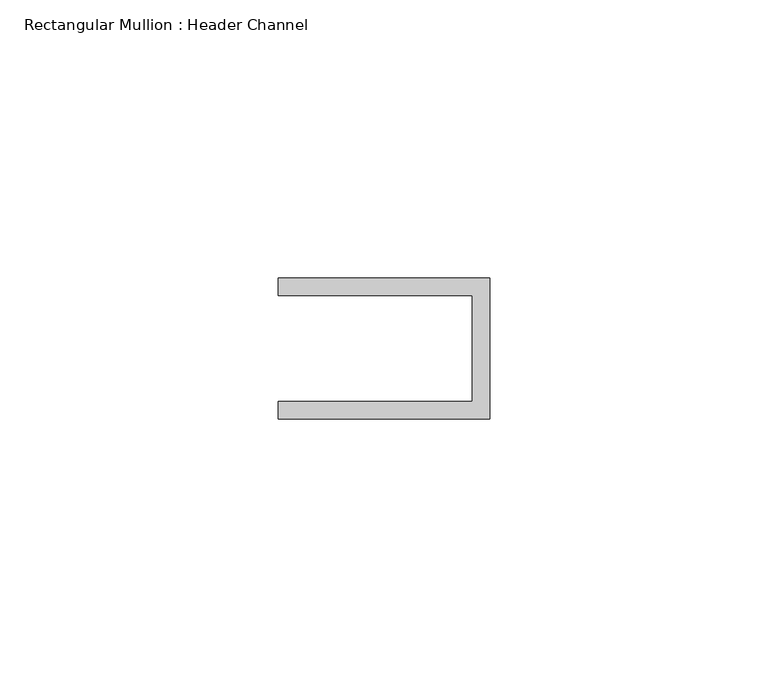
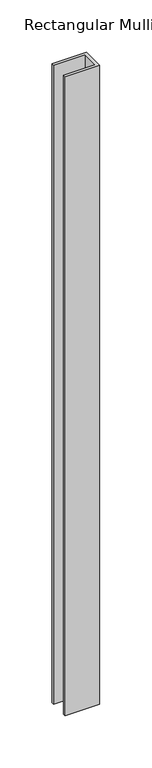
"""IFC4 building model written with IfcOpenShell, lengths in millimetres: member geometry, Rectangular Mullion : Header Channel."""

import ifcopenshell
import ifcopenshell.guid

model = None  # the IFC model being written
_history = None  # IfcOwnerHistory: only IFC2X3 demands one
_inside = {}  # id of a spatial element -> (the spatial element, [elements in it])
_under = {}  # id of a project, library or spatial element -> (it, [spatial elements below it])
_declared = {}  # id of a project -> (the project, [libraries it declares])
_typed = {}  # id of a type object -> (the type object, [elements of that type])
_made_of = {}  # id of a material, layer set ... -> (it, [elements and type objects made of it])


def new_model(schema):
    """Start an empty IFC model of exactly this schema.

    Asked for "IFC4X3", IfcOpenShell would pick the latest addendum, in which some entities
    have other attributes; the version numbers below select the first issue.
    IFC2X3 requires an IfcOwnerHistory on every rooted entity: one is made here for all.
    """
    global model, _history
    if schema == "IFC4X3":
        model = ifcopenshell.file(schema_version=(4, 3, 0, 0))
    else:
        model = ifcopenshell.file(schema=schema)
    _inside.clear()
    _under.clear()
    _declared.clear()
    _typed.clear()
    _made_of.clear()
    _history = None
    if model.schema == "IFC2X3":
        org = make("IfcOrganization", Name="unknown")
        user = make(
            "IfcPersonAndOrganization",
            ThePerson=make("IfcPerson", FamilyName="unknown"),
            TheOrganization=org,
        )
        app = make(
            "IfcApplication",
            ApplicationDeveloper=org,
            Version="unknown",
            ApplicationFullName="unknown",
            ApplicationIdentifier="unknown",
        )
        _history = make(
            "IfcOwnerHistory",
            OwningUser=user,
            OwningApplication=app,
            ChangeAction="ADDED",
            CreationDate=0,
        )
    return model


def make(cls, **values):
    """One entity of the class cls with the attributes given. An attribute that is None is left unset."""
    return model.create_entity(
        cls, **{name: value for name, value in values.items() if value is not None}
    )


def rooted(cls, **values):
    """An entity with a GlobalId (a new one), such as an element, a storey or a relation."""
    return make(cls, GlobalId=ifcopenshell.guid.new(), OwnerHistory=_history, **values)


def si_unit(unit_type, name, prefix=None):
    """IfcSIUnit, for example si_unit("LENGTHUNIT", "METRE", prefix="MILLI")."""
    return make("IfcSIUnit", UnitType=unit_type, Prefix=prefix, Name=name)


def assignment(units):
    """IfcUnitAssignment: the units of a project."""
    return None if units is None else make("IfcUnitAssignment", Units=units)


def point(xyz):
    """IfcCartesianPoint."""
    return None if xyz is None else make("IfcCartesianPoint", Coordinates=xyz)


def direction(xyz):
    """IfcDirection."""
    return None if xyz is None else make("IfcDirection", DirectionRatios=xyz)


def frame(location, z_axis=None, x_axis=None):
    """IfcAxis2Placement3D, a coordinate frame: its origin and axes. An axis left out is left unset."""
    return make(
        "IfcAxis2Placement3D",
        Location=point(location),
        Axis=direction(z_axis),
        RefDirection=direction(x_axis),
    )


def origin():
    """The frame at (0, 0, 0) with its axes left unset."""
    return frame((0.0, 0.0, 0.0))


def place(relative_to, where):
    """IfcLocalPlacement: puts the frame where relative to a parent placement (None: the world)."""
    return make(
        "IfcLocalPlacement", PlacementRelTo=relative_to, RelativePlacement=where
    )


def context(
    kind, dimensions, precision=None, world=None, true_north=None, identifier=None
):
    """IfcGeometricRepresentationContext, for example the 3D "Model" context."""
    return make(
        "IfcGeometricRepresentationContext",
        ContextIdentifier=identifier,
        ContextType=kind,
        CoordinateSpaceDimension=dimensions,
        Precision=precision,
        WorldCoordinateSystem=world,
        TrueNorth=true_north,
    )


def project(units=None, contexts=None):
    """IfcProject with its units and contexts."""
    return rooted(
        "IfcProject",
        Name="project",
        RepresentationContexts=contexts,
        UnitsInContext=assignment(units),
    )


def spatial(cls, under=None, at=None, **own):
    """A site, building, storey or space (cls), placed at a placement, below another one or the project."""
    s = rooted(cls, ObjectPlacement=at, **own)
    if under is not None:
        _under.setdefault(under.id(), (under, []))[1].append(s)
    return s


def polyline(points):
    """IfcPolyline through the points."""
    return make("IfcPolyline", Points=[point(p) for p in points])


def outline(outer, holes=None, kind="AREA"):
    """IfcArbitraryClosedProfileDef: a profile drawn as a closed curve; with holes, ...WithVoids."""
    if holes is None:
        return make("IfcArbitraryClosedProfileDef", ProfileType=kind, OuterCurve=outer)
    return make(
        "IfcArbitraryProfileDefWithVoids",
        ProfileType=kind,
        OuterCurve=outer,
        InnerCurves=holes,
    )


def extrude(swept, where, along, depth):
    """IfcExtrudedAreaSolid: the profile swept, set in the frame where, extruded along a direction by depth."""
    return make(
        "IfcExtrudedAreaSolid",
        SweptArea=swept,
        Position=where,
        ExtrudedDirection=direction(along),
        Depth=depth,
    )


def shape(context_of_items, identifier, shape_type, items):
    """IfcShapeRepresentation: the items that make up one representation, for example the "Body"."""
    return make(
        "IfcShapeRepresentation",
        ContextOfItems=context_of_items,
        RepresentationIdentifier=identifier,
        RepresentationType=shape_type,
        Items=items,
    )


def source(mapping_origin, context_of_items, identifier, shape_type, items):
    """IfcRepresentationMap: a shape defined once, which mapped items show again and again."""
    return make(
        "IfcRepresentationMap",
        MappingOrigin=mapping_origin,
        MappedRepresentation=shape(context_of_items, identifier, shape_type, items),
    )


def transform(
    local_origin,
    x_axis=None,
    y_axis=None,
    z_axis=None,
    scale=None,
    scale2=None,
    scale3=None,
    uniform=True,
):
    """IfcCartesianTransformationOperator3D, or its non-uniform kind. x_axis, y_axis, z_axis: its Axis1, 2, 3."""
    if uniform:
        return make(
            "IfcCartesianTransformationOperator3D",
            Axis1=direction(x_axis),
            Axis2=direction(y_axis),
            LocalOrigin=point(local_origin),
            Scale=scale,
            Axis3=direction(z_axis),
        )
    return make(
        "IfcCartesianTransformationOperator3DnonUniform",
        Axis1=direction(x_axis),
        Axis2=direction(y_axis),
        LocalOrigin=point(local_origin),
        Scale=scale,
        Axis3=direction(z_axis),
        Scale2=scale2,
        Scale3=scale3,
    )


def mapped(mapping_source, mapping_target):
    """IfcMappedItem: shows the shape of a source again, moved by a transform."""
    return make(
        "IfcMappedItem", MappingSource=mapping_source, MappingTarget=mapping_target
    )


def made_of(thing, what):
    """Note that an element or type object is made of a material, layer set ...; save() writes the relation."""
    if what is not None:
        _made_of.setdefault(what.id(), (what, []))[1].append(thing)
    return thing


def element(
    cls,
    number,
    at=None,
    inside=None,
    cuts=None,
    type_object=None,
    material=None,
    context=None,
    identifier="Body",
    shape_type=None,
    held_by="IfcProductDefinitionShape",
    body=None,
    shapes=None,
    **own,
):
    """One element of the class cls, such as IfcWall. Its Tag is "e" and its number.

    at: its placement. inside: the storey or other place that contains it. cuts: it is an
    opening in that element (IfcRelVoidsElement). A single representation is given by context,
    identifier, shape_type and body (its items); several are given by shapes. held_by: the class
    of the entity that holds the representations. save() writes the other relations.
    """
    e = rooted(cls, Tag="e%d" % number, ObjectPlacement=at, **own)
    if body is not None:
        shapes = [shape(context, identifier, shape_type, body)]
    if shapes is not None:
        e.Representation = make(held_by, Representations=shapes)
    if inside is not None:
        _inside.setdefault(inside.id(), (inside, []))[1].append(e)
    if cuts is not None:
        rooted(
            "IfcRelVoidsElement", RelatingBuildingElement=cuts, RelatedOpeningElement=e
        )
    if type_object is not None:
        _typed.setdefault(type_object.id(), (type_object, []))[1].append(e)
    return made_of(e, material)


def aggregate(whole, parts):
    """IfcRelAggregates: a whole, such as a stair, and the parts it consists of."""
    return rooted("IfcRelAggregates", RelatingObject=whole, RelatedObjects=parts)


def save(model, path):
    """Write the relations noted so far, then the file.

    IfcRelAggregates (storeys below a building ...), IfcRelContainedInSpatialStructure (elements
    in a storey), IfcRelDefinesByType, IfcRelAssociatesMaterial and IfcRelDeclares: one each for
    every whole, place, type object, material and project.
    """
    for whole, parts in _under.values():
        aggregate(whole, parts)
    for where, things in _inside.values():
        rooted(
            "IfcRelContainedInSpatialStructure",
            RelatedElements=things,
            RelatingStructure=where,
        )
    for kind, things in _typed.values():
        rooted("IfcRelDefinesByType", RelatedObjects=things, RelatingType=kind)
    for what, things in _made_of.values():
        rooted("IfcRelAssociatesMaterial", RelatedObjects=things, RelatingMaterial=what)
    for by, libraries in _declared.values():
        rooted("IfcRelDeclares", RelatingContext=by, RelatedDefinitions=libraries)
    model.write(path)


def rectangular_mullion_header_channel_9bb2e47f(model_context):
    return source(origin(), model_context, "Body", "SweptSolid", [
        extrude(outline(polyline([(0.0, -12.7), (-38.1, -12.7), (-38.1, -9.525), (-3.175, -9.525), (-3.175, 9.525), (-38.1, 9.525), (-38.1, 12.7), (0.0, 12.7), (0.0, -12.7)])), frame((0.0, 0.0, -747.199643), z_axis=(0.0, 0.0, 1.0), x_axis=(1.0, 0.0, 0.0)), (0.0, 0.0, 1.0), 747.199643),
    ])


if __name__ == "__main__":
    model = new_model("IFC4")
    model_context = context("Model", 3, world=origin())
    ifc_project = project(units=[si_unit("LENGTHUNIT", "METRE", prefix="MILLI")], contexts=[model_context])
    site = spatial("IfcSite", under=ifc_project)
    building = spatial("IfcBuilding", under=site)
    placement = place(None, origin())
    rectangular_mullion_header_channel_shape = rectangular_mullion_header_channel_9bb2e47f(model_context)
    element("IfcMember", 1, ObjectType="Rectangular Mullion : Header Channel", at=placement, inside=building, context=model_context, shape_type="MappedRepresentation", body=[
        mapped(rectangular_mullion_header_channel_shape, transform((0.0, 0.0, 0.0), x_axis=(1.0, 0.0, 0.0), y_axis=(0.0, 1.0, 0.0), z_axis=(0.0, 0.0, 1.0))),
    ])
    save(model, "model.ifc")

# Revit data of these elements
# Type "Rectangular Mullion : Header Channel"
#   built-in parameter 1007322 = 0.0833333 (stored number, unit not read)
#   built-in parameter 1007321 = -0.03125 (stored number, unit not read)
#   built-in parameter 1007320 = 0.0416667 (stored number, unit not read)
# Element 1 (IfcMember, "Rectangular Mullion : Header Channel")
#   Materials on its faces: "ALUM"
# Materials
#   "ALUM": class "Generic", colour RGB 157 157 157, transparency 0, Cost = 0
